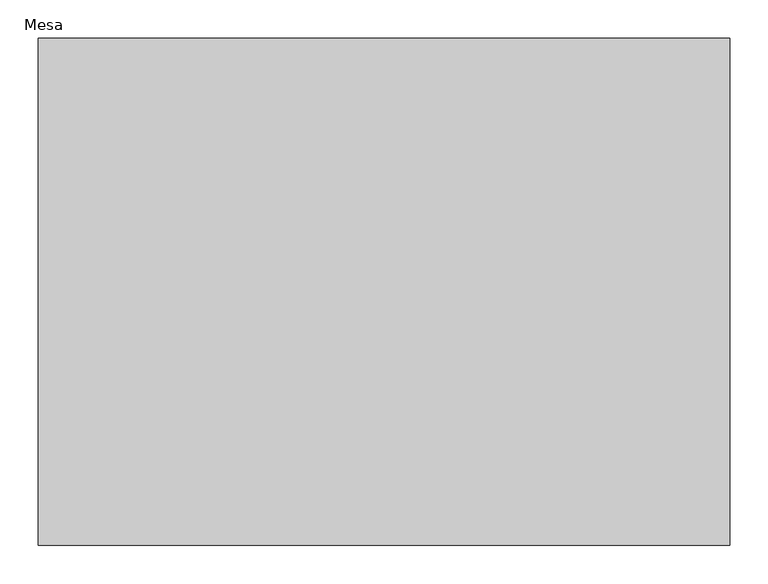
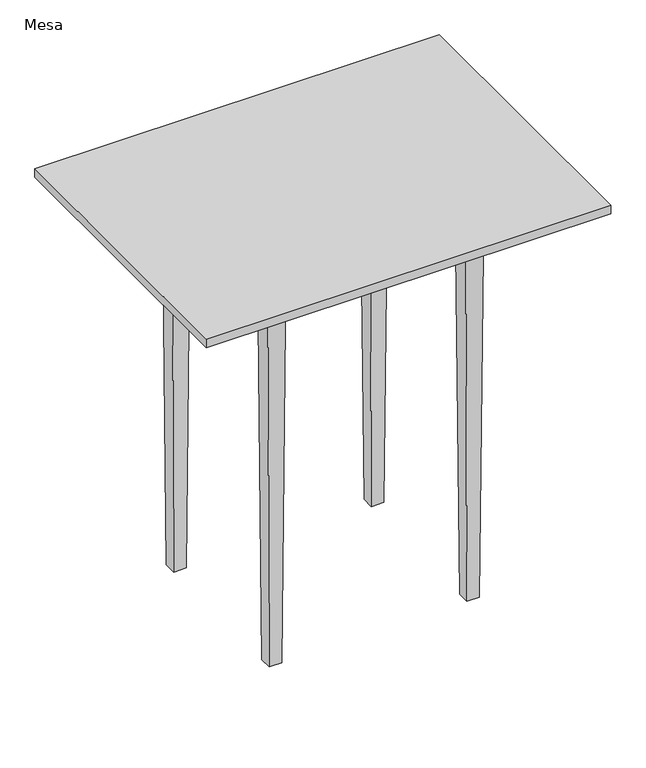
"""IFC4 building model written with IfcOpenShell, lengths in millimetres: furniture geometry, Mesa : Cerrado - 900 x 660 mm."""

from ifc_helpers import new_model, si_unit, frame, origin, place, context, project, spatial, polyline, outline, extrude, faceted_brep, source, transform, mapped, element, save


def mesa_1afdadff(model_context):
    return source(origin(), model_context, "Body", "SolidModel", [
        extrude(outline(polyline([(450.0, 330.0), (450.0, -330.0), (-450.0, -330.0), (-450.0, 330.0), (450.0, 330.0)])), frame((0.0, 0.0, 906.8493799), z_axis=(0.0, 0.0, 1.0), x_axis=(1.0, 0.0, 0.0)), (0.0, 0.0, 1.0), 20.0),
        extrude(outline(polyline([(217.5, 164.0), (232.5, 164.0), (232.5, -163.0212689), (217.5, -163.0212689), (217.5, 164.0)])), frame((0.0, 0.0, 846.8493799), z_axis=(0.0, 0.0, 1.0), x_axis=(1.0, 0.0, 0.0)), (0.0, 0.0, 1.0), 60.0),
        extrude(outline(polyline([(-217.5, 164.0), (-217.5, -163.0212689), (-232.5, -163.0212689), (-232.5, 164.0), (-217.5, 164.0)])), frame((0.0, 0.0, 846.8493799), z_axis=(0.0, 0.0, 1.0), x_axis=(1.0, 0.0, 0.0)), (0.0, 0.0, 1.0), 60.0),
        extrude(outline(polyline([(200.0, -191.1183971), (-200.0, -191.1183971), (-200.0, -176.1183971), (200.0, -176.1183971), (200.0, -191.1183971)])), frame((0.0, 0.0, 846.8493799), z_axis=(0.0, 0.0, 1.0), x_axis=(1.0, 0.0, 0.0)), (0.0, 0.0, 1.0), 60.0),
        extrude(outline(polyline([(200.0, 191.1183971), (200.0, 176.1183971), (-200.0, 176.1183971), (-200.0, 191.1183971), (200.0, 191.1183971)])), frame((0.0, 0.0, 846.8493799), z_axis=(0.0, 0.0, 1.0), x_axis=(1.0, 0.0, 0.0)), (0.0, 0.0, 1.0), 60.0),
        faceted_brep([(200.0, -204.0, 906.8493799), (240.0, -204.0, 906.8493799), (240.0, -164.0, 906.8493799), (200.0, -164.0, 906.8493799), (206.0253573, -198.0, 0.0), (206.0253573, -170.0, 0.0), (234.0253573, -170.0, 0.0), (234.0253573, -198.0, 0.0)], [[[0, 1, 2, 3]], [[4, 5, 6, 7]], [[4, 7, 1, 0]], [[7, 6, 2, 1]], [[6, 5, 3, 2]], [[5, 4, 0, 3]]]),
        faceted_brep([(-200.0, -204.0, 906.8493799), (-200.0, -164.0, 906.8493799), (-240.0, -164.0, 906.8493799), (-240.0, -204.0, 906.8493799), (-206.0253573, -198.0, 0.0), (-234.0253573, -198.0, 0.0), (-234.0253573, -170.0, 0.0), (-206.0253573, -170.0, 0.0)], [[[0, 1, 2, 3]], [[4, 5, 6, 7]], [[4, 7, 1, 0]], [[7, 6, 2, 1]], [[6, 5, 3, 2]], [[5, 4, 0, 3]]]),
        faceted_brep([(200.0, 204.0, 906.8493799), (200.0, 164.0, 906.8493799), (240.0, 164.0, 906.8493799), (240.0, 204.0, 906.8493799), (206.0253573, 198.0, 0.0), (234.0253573, 198.0, 0.0), (234.0253573, 170.0, 0.0), (206.0253573, 170.0, 0.0)], [[[0, 1, 2, 3]], [[4, 5, 6, 7]], [[4, 7, 1, 0]], [[7, 6, 2, 1]], [[6, 5, 3, 2]], [[5, 4, 0, 3]]]),
        faceted_brep([(-200.0, 204.0, 906.8493799), (-240.0, 204.0, 906.8493799), (-240.0, 164.0, 906.8493799), (-200.0, 164.0, 906.8493799), (-206.0253573, 198.0, 0.0), (-206.0253573, 170.0, 0.0), (-234.0253573, 170.0, 0.0), (-234.0253573, 198.0, 0.0)], [[[0, 1, 2, 3]], [[4, 5, 6, 7]], [[4, 7, 1, 0]], [[7, 6, 2, 1]], [[6, 5, 3, 2]], [[5, 4, 0, 3]]]),
    ])


if __name__ == "__main__":
    model = new_model("IFC4")
    model_context = context("Model", 3, world=origin())
    ifc_project = project(units=[si_unit("LENGTHUNIT", "METRE", prefix="MILLI")], contexts=[model_context])
    site = spatial("IfcSite", under=ifc_project)
    building = spatial("IfcBuilding", under=site)
    placement = place(None, origin())
    mesa_shape = mesa_1afdadff(model_context)
    element("IfcFurniture", 1, ObjectType="Mesa : Cerrado - 900 x 660 mm", at=placement, inside=building, context=model_context, shape_type="MappedRepresentation", body=[
        mapped(mesa_shape, transform((0.0, 0.0, 0.0), x_axis=(1.0, 0.0, 0.0), y_axis=(0.0, 1.0, 0.0), z_axis=(0.0, 0.0, 1.0))),
    ])
    save(model, "model.ifc")

# Revit data of these elements
# Type "Mesa : Cerrado - 900 x 660 mm"
#   Anchura = 0.90 m
#   Altura = 0.926849 m
#   Profundidad = 0.66 m
#   Máscara [instance default] = yes
#   Material = none
#   Default Elevation = 0
#   Manufacturer = ""
# Element 1 (IfcFurniture, "Mesa : Cerrado - 900 x 660 mm")
#   Materials on its faces: "Madera - Listel"
# Materials
#   "Madera - Listel": class "Madera", colour RGB 210 180 110, transparency 0, Cost = 0
